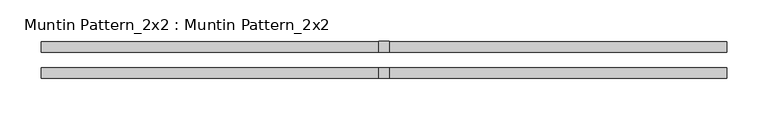
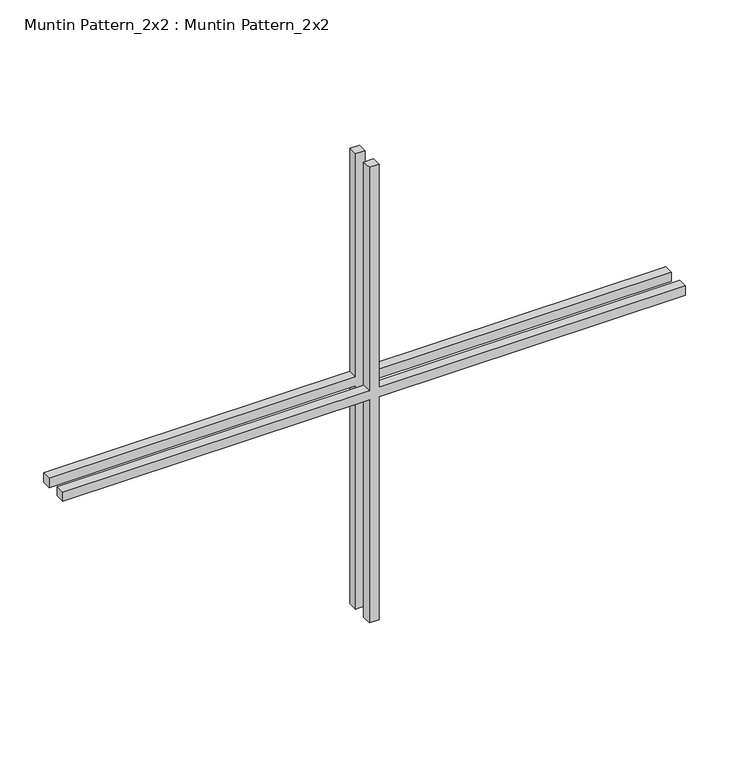
"""IFC4 building model written with IfcOpenShell, lengths in millimetres: proxy geometry, Muntin Pattern_2x2 : Muntin Pattern_2x2."""

import ifcopenshell
import ifcopenshell.guid

model = None  # the IFC model being written
_history = None  # IfcOwnerHistory: only IFC2X3 demands one
_inside = {}  # id of a spatial element -> (the spatial element, [elements in it])
_under = {}  # id of a project, library or spatial element -> (it, [spatial elements below it])
_declared = {}  # id of a project -> (the project, [libraries it declares])
_typed = {}  # id of a type object -> (the type object, [elements of that type])
_made_of = {}  # id of a material, layer set ... -> (it, [elements and type objects made of it])


def new_model(schema):
    """Start an empty IFC model of exactly this schema.

    Asked for "IFC4X3", IfcOpenShell would pick the latest addendum, in which some entities
    have other attributes; the version numbers below select the first issue.
    IFC2X3 requires an IfcOwnerHistory on every rooted entity: one is made here for all.
    """
    global model, _history
    if schema == "IFC4X3":
        model = ifcopenshell.file(schema_version=(4, 3, 0, 0))
    else:
        model = ifcopenshell.file(schema=schema)
    _inside.clear()
    _under.clear()
    _declared.clear()
    _typed.clear()
    _made_of.clear()
    _history = None
    if model.schema == "IFC2X3":
        org = make("IfcOrganization", Name="unknown")
        user = make(
            "IfcPersonAndOrganization",
            ThePerson=make("IfcPerson", FamilyName="unknown"),
            TheOrganization=org,
        )
        app = make(
            "IfcApplication",
            ApplicationDeveloper=org,
            Version="unknown",
            ApplicationFullName="unknown",
            ApplicationIdentifier="unknown",
        )
        _history = make(
            "IfcOwnerHistory",
            OwningUser=user,
            OwningApplication=app,
            ChangeAction="ADDED",
            CreationDate=0,
        )
    return model


def make(cls, **values):
    """One entity of the class cls with the attributes given. An attribute that is None is left unset."""
    return model.create_entity(
        cls, **{name: value for name, value in values.items() if value is not None}
    )


def rooted(cls, **values):
    """An entity with a GlobalId (a new one), such as an element, a storey or a relation."""
    return make(cls, GlobalId=ifcopenshell.guid.new(), OwnerHistory=_history, **values)


def si_unit(unit_type, name, prefix=None):
    """IfcSIUnit, for example si_unit("LENGTHUNIT", "METRE", prefix="MILLI")."""
    return make("IfcSIUnit", UnitType=unit_type, Prefix=prefix, Name=name)


def assignment(units):
    """IfcUnitAssignment: the units of a project."""
    return None if units is None else make("IfcUnitAssignment", Units=units)


def point(xyz):
    """IfcCartesianPoint."""
    return None if xyz is None else make("IfcCartesianPoint", Coordinates=xyz)


def direction(xyz):
    """IfcDirection."""
    return None if xyz is None else make("IfcDirection", DirectionRatios=xyz)


def frame(location, z_axis=None, x_axis=None):
    """IfcAxis2Placement3D, a coordinate frame: its origin and axes. An axis left out is left unset."""
    return make(
        "IfcAxis2Placement3D",
        Location=point(location),
        Axis=direction(z_axis),
        RefDirection=direction(x_axis),
    )


def origin():
    """The frame at (0, 0, 0) with its axes left unset."""
    return frame((0.0, 0.0, 0.0))


def place(relative_to, where):
    """IfcLocalPlacement: puts the frame where relative to a parent placement (None: the world)."""
    return make(
        "IfcLocalPlacement", PlacementRelTo=relative_to, RelativePlacement=where
    )


def context(
    kind, dimensions, precision=None, world=None, true_north=None, identifier=None
):
    """IfcGeometricRepresentationContext, for example the 3D "Model" context."""
    return make(
        "IfcGeometricRepresentationContext",
        ContextIdentifier=identifier,
        ContextType=kind,
        CoordinateSpaceDimension=dimensions,
        Precision=precision,
        WorldCoordinateSystem=world,
        TrueNorth=true_north,
    )


def project(units=None, contexts=None):
    """IfcProject with its units and contexts."""
    return rooted(
        "IfcProject",
        Name="project",
        RepresentationContexts=contexts,
        UnitsInContext=assignment(units),
    )


def spatial(cls, under=None, at=None, **own):
    """A site, building, storey or space (cls), placed at a placement, below another one or the project."""
    s = rooted(cls, ObjectPlacement=at, **own)
    if under is not None:
        _under.setdefault(under.id(), (under, []))[1].append(s)
    return s


def polyline(points):
    """IfcPolyline through the points."""
    return make("IfcPolyline", Points=[point(p) for p in points])


def outline(outer, holes=None, kind="AREA"):
    """IfcArbitraryClosedProfileDef: a profile drawn as a closed curve; with holes, ...WithVoids."""
    if holes is None:
        return make("IfcArbitraryClosedProfileDef", ProfileType=kind, OuterCurve=outer)
    return make(
        "IfcArbitraryProfileDefWithVoids",
        ProfileType=kind,
        OuterCurve=outer,
        InnerCurves=holes,
    )


def extrude(swept, where, along, depth):
    """IfcExtrudedAreaSolid: the profile swept, set in the frame where, extruded along a direction by depth."""
    return make(
        "IfcExtrudedAreaSolid",
        SweptArea=swept,
        Position=where,
        ExtrudedDirection=direction(along),
        Depth=depth,
    )


def shape(context_of_items, identifier, shape_type, items):
    """IfcShapeRepresentation: the items that make up one representation, for example the "Body"."""
    return make(
        "IfcShapeRepresentation",
        ContextOfItems=context_of_items,
        RepresentationIdentifier=identifier,
        RepresentationType=shape_type,
        Items=items,
    )


def source(mapping_origin, context_of_items, identifier, shape_type, items):
    """IfcRepresentationMap: a shape defined once, which mapped items show again and again."""
    return make(
        "IfcRepresentationMap",
        MappingOrigin=mapping_origin,
        MappedRepresentation=shape(context_of_items, identifier, shape_type, items),
    )


def transform(
    local_origin,
    x_axis=None,
    y_axis=None,
    z_axis=None,
    scale=None,
    scale2=None,
    scale3=None,
    uniform=True,
):
    """IfcCartesianTransformationOperator3D, or its non-uniform kind. x_axis, y_axis, z_axis: its Axis1, 2, 3."""
    if uniform:
        return make(
            "IfcCartesianTransformationOperator3D",
            Axis1=direction(x_axis),
            Axis2=direction(y_axis),
            LocalOrigin=point(local_origin),
            Scale=scale,
            Axis3=direction(z_axis),
        )
    return make(
        "IfcCartesianTransformationOperator3DnonUniform",
        Axis1=direction(x_axis),
        Axis2=direction(y_axis),
        LocalOrigin=point(local_origin),
        Scale=scale,
        Axis3=direction(z_axis),
        Scale2=scale2,
        Scale3=scale3,
    )


def mapped(mapping_source, mapping_target):
    """IfcMappedItem: shows the shape of a source again, moved by a transform."""
    return make(
        "IfcMappedItem", MappingSource=mapping_source, MappingTarget=mapping_target
    )


def made_of(thing, what):
    """Note that an element or type object is made of a material, layer set ...; save() writes the relation."""
    if what is not None:
        _made_of.setdefault(what.id(), (what, []))[1].append(thing)
    return thing


def element(
    cls,
    number,
    at=None,
    inside=None,
    cuts=None,
    type_object=None,
    material=None,
    context=None,
    identifier="Body",
    shape_type=None,
    held_by="IfcProductDefinitionShape",
    body=None,
    shapes=None,
    **own,
):
    """One element of the class cls, such as IfcWall. Its Tag is "e" and its number.

    at: its placement. inside: the storey or other place that contains it. cuts: it is an
    opening in that element (IfcRelVoidsElement). A single representation is given by context,
    identifier, shape_type and body (its items); several are given by shapes. held_by: the class
    of the entity that holds the representations. save() writes the other relations.
    """
    e = rooted(cls, Tag="e%d" % number, ObjectPlacement=at, **own)
    if body is not None:
        shapes = [shape(context, identifier, shape_type, body)]
    if shapes is not None:
        e.Representation = make(held_by, Representations=shapes)
    if inside is not None:
        _inside.setdefault(inside.id(), (inside, []))[1].append(e)
    if cuts is not None:
        rooted(
            "IfcRelVoidsElement", RelatingBuildingElement=cuts, RelatedOpeningElement=e
        )
    if type_object is not None:
        _typed.setdefault(type_object.id(), (type_object, []))[1].append(e)
    return made_of(e, material)


def aggregate(whole, parts):
    """IfcRelAggregates: a whole, such as a stair, and the parts it consists of."""
    return rooted("IfcRelAggregates", RelatingObject=whole, RelatedObjects=parts)


def save(model, path):
    """Write the relations noted so far, then the file.

    IfcRelAggregates (storeys below a building ...), IfcRelContainedInSpatialStructure (elements
    in a storey), IfcRelDefinesByType, IfcRelAssociatesMaterial and IfcRelDeclares: one each for
    every whole, place, type object, material and project.
    """
    for whole, parts in _under.values():
        aggregate(whole, parts)
    for where, things in _inside.values():
        rooted(
            "IfcRelContainedInSpatialStructure",
            RelatedElements=things,
            RelatingStructure=where,
        )
    for kind, things in _typed.values():
        rooted("IfcRelDefinesByType", RelatedObjects=things, RelatingType=kind)
    for what, things in _made_of.values():
        rooted("IfcRelAssociatesMaterial", RelatedObjects=things, RelatingMaterial=what)
    for by, libraries in _declared.values():
        rooted("IfcRelDeclares", RelatingContext=by, RelatedDefinitions=libraries)
    model.write(path)


def muntin_pattern_2x2_muntin_pattern_2x2_6dda0405(model_context):
    return source(origin(), model_context, "Body", "SweptSolid", [
        extrude(outline(polyline([(325.4375, -6.35), (325.4375, -412.75), (312.7375, -412.75), (312.7375, -6.35), (0.0, -6.35), (0.0, 6.35), (312.7375, 6.35), (312.7375, 412.75), (325.4375, 412.75), (325.4375, 6.35), (638.175, 6.35), (638.175, -6.35), (325.4375, -6.35)])), frame((0.0, 9.525, 0.0), z_axis=(0.0, 1.0, 0.0), x_axis=(0.0, 0.0, 1.0)), (0.0, 0.0, 1.0), 12.7),
        extrude(outline(polyline([(325.4375, -6.35), (325.4375, -412.75), (312.7375, -412.75), (312.7375, -6.35), (0.0, -6.35), (0.0, 6.35), (312.7375, 6.35), (312.7375, 412.75), (325.4375, 412.75), (325.4375, 6.35), (638.175, 6.35), (638.175, -6.35), (325.4375, -6.35)])), frame((0.0, -22.225, 0.0), z_axis=(0.0, 1.0, 0.0), x_axis=(0.0, 0.0, 1.0)), (0.0, 0.0, 1.0), 12.7),
    ])


if __name__ == "__main__":
    model = new_model("IFC4")
    model_context = context("Model", 3, world=origin())
    ifc_project = project(units=[si_unit("LENGTHUNIT", "METRE", prefix="MILLI")], contexts=[model_context])
    site = spatial("IfcSite", under=ifc_project)
    building = spatial("IfcBuilding", under=site)
    placement = place(None, origin())
    muntin_pattern_2x2_muntin_pattern_2x2_shape = muntin_pattern_2x2_muntin_pattern_2x2_6dda0405(model_context)
    element("IfcBuildingElementProxy", 1, Name="Muntin Pattern_2x2 : Muntin Pattern_2x2", ObjectType="Muntin Pattern_2x2 : Muntin Pattern_2x2", at=placement, inside=building, context=model_context, shape_type="MappedRepresentation", body=[
        mapped(muntin_pattern_2x2_muntin_pattern_2x2_shape, transform((0.0, 0.0, 0.0), x_axis=(1.0, 0.0, 0.0), y_axis=(0.0, 1.0, 0.0), z_axis=(0.0, 0.0, 1.0))),
    ])
    save(model, "model.ifc")

# Revit data of these elements
# Type "Muntin Pattern_2x2 : Muntin Pattern_2x2"
#   Width [instance default] = 4' - 0"
#   Thickness = 0' - 0 1/2"
#   Height [instance default] = 4' - 0"
#   Distance = 0' - 0 3/4"
#   Interior Material [instance default] = none
#   Exterior Material [instance default] = none
# Element 1 (IfcBuildingElementProxy, "Muntin Pattern_2x2 : Muntin Pattern_2x2")
#   Width = 2' - 8 1/2"
#   Height = 2' - 1 1/8"
#   Interior Material = Wood - Stained
#   Exterior Material = Clad - White
#   Materials on its faces: "Clad - White", "Wood - Stained"
# Materials
#   "Clad - White": class "Wood", colour RGB 242 242 238, transparency 0, Cost = 0
#   "Wood - Stained": class "Wood", colour RGB 224 178 126, transparency 0, Cost = 0
